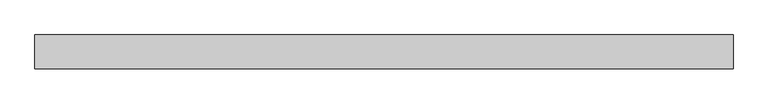
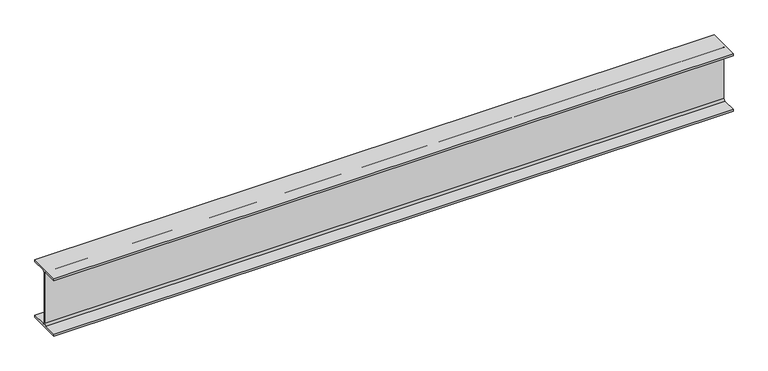
"""IFC4 building model written with IfcOpenShell, lengths in millimetres: beam geometry, Steel Beam_H-KSD3502 : H_SB_ASB_H-200x200x8x12."""

import ifcopenshell
import ifcopenshell.guid

model = None  # the IFC model being written
_history = None  # IfcOwnerHistory: only IFC2X3 demands one
_inside = {}  # id of a spatial element -> (the spatial element, [elements in it])
_under = {}  # id of a project, library or spatial element -> (it, [spatial elements below it])
_declared = {}  # id of a project -> (the project, [libraries it declares])
_typed = {}  # id of a type object -> (the type object, [elements of that type])
_made_of = {}  # id of a material, layer set ... -> (it, [elements and type objects made of it])


def new_model(schema):
    """Start an empty IFC model of exactly this schema.

    Asked for "IFC4X3", IfcOpenShell would pick the latest addendum, in which some entities
    have other attributes; the version numbers below select the first issue.
    IFC2X3 requires an IfcOwnerHistory on every rooted entity: one is made here for all.
    """
    global model, _history
    if schema == "IFC4X3":
        model = ifcopenshell.file(schema_version=(4, 3, 0, 0))
    else:
        model = ifcopenshell.file(schema=schema)
    _inside.clear()
    _under.clear()
    _declared.clear()
    _typed.clear()
    _made_of.clear()
    _history = None
    if model.schema == "IFC2X3":
        org = make("IfcOrganization", Name="unknown")
        user = make(
            "IfcPersonAndOrganization",
            ThePerson=make("IfcPerson", FamilyName="unknown"),
            TheOrganization=org,
        )
        app = make(
            "IfcApplication",
            ApplicationDeveloper=org,
            Version="unknown",
            ApplicationFullName="unknown",
            ApplicationIdentifier="unknown",
        )
        _history = make(
            "IfcOwnerHistory",
            OwningUser=user,
            OwningApplication=app,
            ChangeAction="ADDED",
            CreationDate=0,
        )
    return model


def make(cls, **values):
    """One entity of the class cls with the attributes given. An attribute that is None is left unset."""
    return model.create_entity(
        cls, **{name: value for name, value in values.items() if value is not None}
    )


def rooted(cls, **values):
    """An entity with a GlobalId (a new one), such as an element, a storey or a relation."""
    return make(cls, GlobalId=ifcopenshell.guid.new(), OwnerHistory=_history, **values)


def si_unit(unit_type, name, prefix=None):
    """IfcSIUnit, for example si_unit("LENGTHUNIT", "METRE", prefix="MILLI")."""
    return make("IfcSIUnit", UnitType=unit_type, Prefix=prefix, Name=name)


def assignment(units):
    """IfcUnitAssignment: the units of a project."""
    return None if units is None else make("IfcUnitAssignment", Units=units)


def point(xyz):
    """IfcCartesianPoint."""
    return None if xyz is None else make("IfcCartesianPoint", Coordinates=xyz)


def direction(xyz):
    """IfcDirection."""
    return None if xyz is None else make("IfcDirection", DirectionRatios=xyz)


def frame(location, z_axis=None, x_axis=None):
    """IfcAxis2Placement3D, a coordinate frame: its origin and axes. An axis left out is left unset."""
    return make(
        "IfcAxis2Placement3D",
        Location=point(location),
        Axis=direction(z_axis),
        RefDirection=direction(x_axis),
    )


def frame_2d(location, x_axis=None):
    """IfcAxis2Placement2D, a coordinate frame in the plane: its origin and x axis."""
    return make(
        "IfcAxis2Placement2D", Location=point(location), RefDirection=direction(x_axis)
    )


def origin():
    """The frame at (0, 0, 0) with its axes left unset."""
    return frame((0.0, 0.0, 0.0))


def place(relative_to, where):
    """IfcLocalPlacement: puts the frame where relative to a parent placement (None: the world)."""
    return make(
        "IfcLocalPlacement", PlacementRelTo=relative_to, RelativePlacement=where
    )


def context(
    kind, dimensions, precision=None, world=None, true_north=None, identifier=None
):
    """IfcGeometricRepresentationContext, for example the 3D "Model" context."""
    return make(
        "IfcGeometricRepresentationContext",
        ContextIdentifier=identifier,
        ContextType=kind,
        CoordinateSpaceDimension=dimensions,
        Precision=precision,
        WorldCoordinateSystem=world,
        TrueNorth=true_north,
    )


def project(units=None, contexts=None):
    """IfcProject with its units and contexts."""
    return rooted(
        "IfcProject",
        Name="project",
        RepresentationContexts=contexts,
        UnitsInContext=assignment(units),
    )


def spatial(cls, under=None, at=None, **own):
    """A site, building, storey or space (cls), placed at a placement, below another one or the project."""
    s = rooted(cls, ObjectPlacement=at, **own)
    if under is not None:
        _under.setdefault(under.id(), (under, []))[1].append(s)
    return s


def polyline(points):
    """IfcPolyline through the points."""
    return make("IfcPolyline", Points=[point(p) for p in points])


def circle_curve(where, radius):
    """IfcCircle in the frame where."""
    return make("IfcCircle", Position=where, Radius=radius)


def trimmed(basis, trim1, trim2, sense, master):
    """IfcTrimmedCurve: the piece of a basis curve between two trims."""
    return make(
        "IfcTrimmedCurve",
        BasisCurve=basis,
        Trim1=trim1,
        Trim2=trim2,
        SenseAgreement=sense,
        MasterRepresentation=master,
    )


def segment(curve, same_sense, transition):
    """IfcCompositeCurveSegment."""
    return make(
        "IfcCompositeCurveSegment",
        Transition=transition,
        SameSense=same_sense,
        ParentCurve=curve,
    )


def composite_curve(segments, self_intersect=None):
    """IfcCompositeCurve: segments joined end to end."""
    return make("IfcCompositeCurve", Segments=segments, SelfIntersect=self_intersect)


def outline(outer, holes=None, kind="AREA"):
    """IfcArbitraryClosedProfileDef: a profile drawn as a closed curve; with holes, ...WithVoids."""
    if holes is None:
        return make("IfcArbitraryClosedProfileDef", ProfileType=kind, OuterCurve=outer)
    return make(
        "IfcArbitraryProfileDefWithVoids",
        ProfileType=kind,
        OuterCurve=outer,
        InnerCurves=holes,
    )


def extrude(swept, where, along, depth):
    """IfcExtrudedAreaSolid: the profile swept, set in the frame where, extruded along a direction by depth."""
    return make(
        "IfcExtrudedAreaSolid",
        SweptArea=swept,
        Position=where,
        ExtrudedDirection=direction(along),
        Depth=depth,
    )


def shape(context_of_items, identifier, shape_type, items):
    """IfcShapeRepresentation: the items that make up one representation, for example the "Body"."""
    return make(
        "IfcShapeRepresentation",
        ContextOfItems=context_of_items,
        RepresentationIdentifier=identifier,
        RepresentationType=shape_type,
        Items=items,
    )


def source(mapping_origin, context_of_items, identifier, shape_type, items):
    """IfcRepresentationMap: a shape defined once, which mapped items show again and again."""
    return make(
        "IfcRepresentationMap",
        MappingOrigin=mapping_origin,
        MappedRepresentation=shape(context_of_items, identifier, shape_type, items),
    )


def transform(
    local_origin,
    x_axis=None,
    y_axis=None,
    z_axis=None,
    scale=None,
    scale2=None,
    scale3=None,
    uniform=True,
):
    """IfcCartesianTransformationOperator3D, or its non-uniform kind. x_axis, y_axis, z_axis: its Axis1, 2, 3."""
    if uniform:
        return make(
            "IfcCartesianTransformationOperator3D",
            Axis1=direction(x_axis),
            Axis2=direction(y_axis),
            LocalOrigin=point(local_origin),
            Scale=scale,
            Axis3=direction(z_axis),
        )
    return make(
        "IfcCartesianTransformationOperator3DnonUniform",
        Axis1=direction(x_axis),
        Axis2=direction(y_axis),
        LocalOrigin=point(local_origin),
        Scale=scale,
        Axis3=direction(z_axis),
        Scale2=scale2,
        Scale3=scale3,
    )


def mapped(mapping_source, mapping_target):
    """IfcMappedItem: shows the shape of a source again, moved by a transform."""
    return make(
        "IfcMappedItem", MappingSource=mapping_source, MappingTarget=mapping_target
    )


def made_of(thing, what):
    """Note that an element or type object is made of a material, layer set ...; save() writes the relation."""
    if what is not None:
        _made_of.setdefault(what.id(), (what, []))[1].append(thing)
    return thing


def element(
    cls,
    number,
    at=None,
    inside=None,
    cuts=None,
    type_object=None,
    material=None,
    context=None,
    identifier="Body",
    shape_type=None,
    held_by="IfcProductDefinitionShape",
    body=None,
    shapes=None,
    **own,
):
    """One element of the class cls, such as IfcWall. Its Tag is "e" and its number.

    at: its placement. inside: the storey or other place that contains it. cuts: it is an
    opening in that element (IfcRelVoidsElement). A single representation is given by context,
    identifier, shape_type and body (its items); several are given by shapes. held_by: the class
    of the entity that holds the representations. save() writes the other relations.
    """
    e = rooted(cls, Tag="e%d" % number, ObjectPlacement=at, **own)
    if body is not None:
        shapes = [shape(context, identifier, shape_type, body)]
    if shapes is not None:
        e.Representation = make(held_by, Representations=shapes)
    if inside is not None:
        _inside.setdefault(inside.id(), (inside, []))[1].append(e)
    if cuts is not None:
        rooted(
            "IfcRelVoidsElement", RelatingBuildingElement=cuts, RelatedOpeningElement=e
        )
    if type_object is not None:
        _typed.setdefault(type_object.id(), (type_object, []))[1].append(e)
    return made_of(e, material)


def aggregate(whole, parts):
    """IfcRelAggregates: a whole, such as a stair, and the parts it consists of."""
    return rooted("IfcRelAggregates", RelatingObject=whole, RelatedObjects=parts)


def save(model, path):
    """Write the relations noted so far, then the file.

    IfcRelAggregates (storeys below a building ...), IfcRelContainedInSpatialStructure (elements
    in a storey), IfcRelDefinesByType, IfcRelAssociatesMaterial and IfcRelDeclares: one each for
    every whole, place, type object, material and project.
    """
    for whole, parts in _under.values():
        aggregate(whole, parts)
    for where, things in _inside.values():
        rooted(
            "IfcRelContainedInSpatialStructure",
            RelatedElements=things,
            RelatingStructure=where,
        )
    for kind, things in _typed.values():
        rooted("IfcRelDefinesByType", RelatedObjects=things, RelatingType=kind)
    for what, things in _made_of.values():
        rooted("IfcRelAssociatesMaterial", RelatedObjects=things, RelatingMaterial=what)
    for by, libraries in _declared.values():
        rooted("IfcRelDeclares", RelatingContext=by, RelatedDefinitions=libraries)
    model.write(path)


def beam_06b2af13(model_context):
    return source(origin(), model_context, "Body", "SweptSolid", [
        extrude(outline(composite_curve([segment(polyline([(82.5, -141.5), (82.5, -151.7), (-82.5, -151.7), (-82.5, -141.5), (-11.9, -141.5)]), True, "CONTINUOUS"), segment(trimmed(circle_curve(frame_2d((-11.9, -132.6)), 8.9), [point((-11.9, -141.5))], [point((-3.0, -132.6))], True, "CARTESIAN"), True, "CONTINUOUS"), segment(polyline([(-3.0, -132.6), (-3.0, 132.6)]), True, "CONTINUOUS"), segment(trimmed(circle_curve(frame_2d((-11.9, 132.6)), 8.9), [point((-3.0, 132.6))], [point((-11.9, 141.5))], True, "CARTESIAN"), True, "CONTINUOUS"), segment(polyline([(-11.9, 141.5), (-82.5, 141.5), (-82.5, 151.7), (82.5, 151.7), (82.5, 141.5), (11.9, 141.5)]), True, "CONTINUOUS"), segment(trimmed(circle_curve(frame_2d((11.9, 132.6)), 8.9), [point((11.9, 141.5))], [point((3.0, 132.6))], True, "CARTESIAN"), True, "CONTINUOUS"), segment(polyline([(3.0, 132.6), (3.0, -132.6)]), True, "CONTINUOUS"), segment(trimmed(circle_curve(frame_2d((11.9, -132.6)), 8.9), [point((3.0, -132.6))], [point((11.9, -141.5))], True, "CARTESIAN"), True, "CONTINUOUS"), segment(polyline([(11.9, -141.5), (82.5, -141.5)]), True, "CONTINUOUS")], self_intersect=False)), frame((-1581.0252804, 0.0, 0.0), z_axis=(1.0, 0.0, 0.0), x_axis=(0.0, 1.0, 0.0)), (0.0, 0.0, 1.0), 3401.4951694),
    ])


if __name__ == "__main__":
    model = new_model("IFC4")
    model_context = context("Model", 3, world=origin())
    ifc_project = project(units=[si_unit("LENGTHUNIT", "METRE", prefix="MILLI")], contexts=[model_context])
    site = spatial("IfcSite", under=ifc_project)
    building = spatial("IfcBuilding", under=site)
    placement = place(None, origin())
    beam_shape = beam_06b2af13(model_context)
    element("IfcBeam", 1, ObjectType="Steel Beam_H-KSD3502 : H_SB_ASB_H-200x200x8x12", at=placement, inside=building, context=model_context, shape_type="MappedRepresentation", body=[
        mapped(beam_shape, transform((0.0, 0.0, 0.0), x_axis=(1.0, 0.0, 0.0), y_axis=(0.0, 1.0, 0.0), z_axis=(0.0, 0.0, 1.0))),
    ])
    save(model, "model.ifc")

# Revit data of these elements
# Project information
#   Building Name = "STEAM TURBINE BUILDING"
#   H_Building Tag = "STB"
#   Project Status = "종결"
#   Client Name = "Therma Viayas Inc.\nTherma Viayas Inc.\nTherma Viayas Inc.\nTherma Viayas Inc."
#   Project Name = "Therma Visayas 2*150MW CFB Power Plant"
#   Project Number = "BEPH1402"
# Type "Steel Beam_H-KSD3502 : H_SB_ASB_H-200x200x8x12"
#   Width = 20.0 cm
#   Web Thickness = 0.8 cm
#   Web Fillet = 1.3 cm
#   Warping Constant = 141376.0 cm⁶
#   Torsional Moment of Inertia = 26.2485 cm⁴
#   Torsional Modulus = 1.0 cm³
#   Section Area = 63.53 cm²
#   Plastic Modulus weak axis = 244.0 cm³
#   Plastic Modulus strong axis = 525.0 cm³
#   Perimeter = 1.16 m²/m
#   Nominal Weight = 49.90 kgf/m
#   Moment of Inertia weak axis = 1600.00 cm⁴
#   Moment of Inertia strong axis = 4720.00 cm⁴
#   Height = 20.0 cm
#   Flange Thickness = 1.2 cm
#   Elastic Modulus weak axis = 160.0 cm³
#   Elastic Modulus strong axis = 472.0 cm³
#   Centroid Vertical = 10.0 cm
#   Centroid Horizontal = 10.0 cm
#   Length [instance default] = 1.5240 m
#   Structural Material [instance default] = Steel, 45-345
#   Assembly Code = ""
# Element 1 (IfcBeam, "Steel Beam_H-KSD3502 : H_SB_ASB_H-200x200x8x12")
#   Structural Material = none
# Materials
#   "Steel, 45-345": class "Metal", colour RGB 189 187 185, transparency 0, Description = "Steel 345 MPa", Cost = 0
